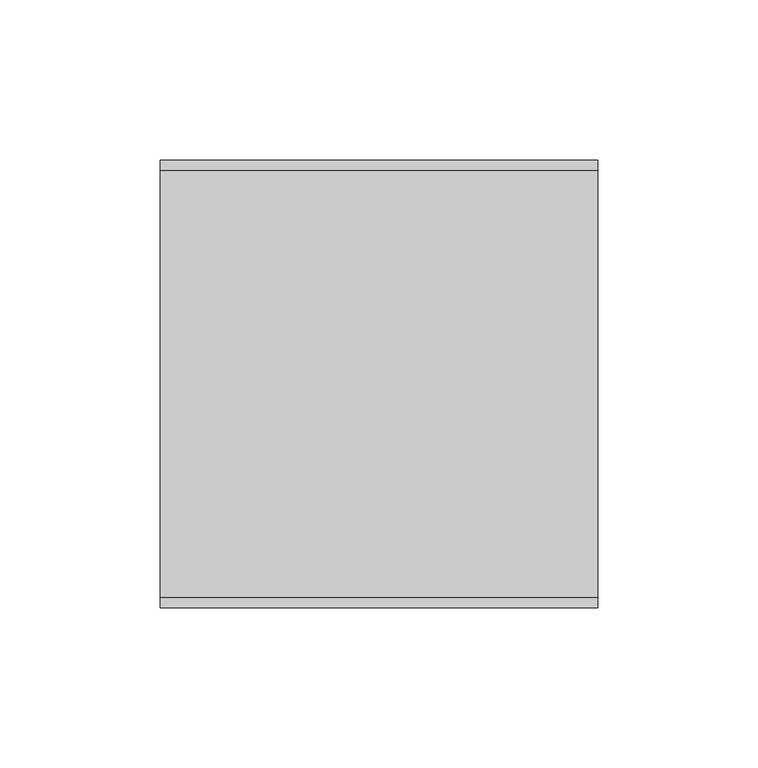
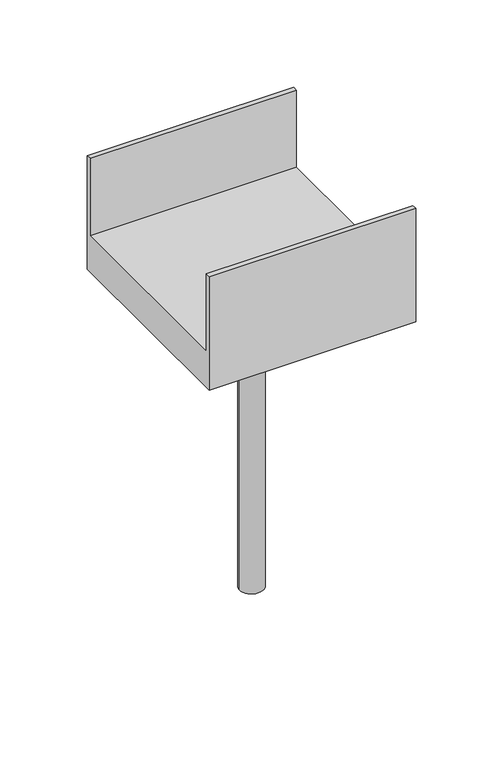
"""IFC4 building model written with IfcOpenShell, lengths in millimetres: fastener geometry."""

import ifcopenshell
import ifcopenshell.guid

model = None  # the IFC model being written
_history = None  # IfcOwnerHistory: only IFC2X3 demands one
_inside = {}  # id of a spatial element -> (the spatial element, [elements in it])
_under = {}  # id of a project, library or spatial element -> (it, [spatial elements below it])
_declared = {}  # id of a project -> (the project, [libraries it declares])
_typed = {}  # id of a type object -> (the type object, [elements of that type])
_made_of = {}  # id of a material, layer set ... -> (it, [elements and type objects made of it])


def new_model(schema):
    """Start an empty IFC model of exactly this schema.

    Asked for "IFC4X3", IfcOpenShell would pick the latest addendum, in which some entities
    have other attributes; the version numbers below select the first issue.
    IFC2X3 requires an IfcOwnerHistory on every rooted entity: one is made here for all.
    """
    global model, _history
    if schema == "IFC4X3":
        model = ifcopenshell.file(schema_version=(4, 3, 0, 0))
    else:
        model = ifcopenshell.file(schema=schema)
    _inside.clear()
    _under.clear()
    _declared.clear()
    _typed.clear()
    _made_of.clear()
    _history = None
    if model.schema == "IFC2X3":
        org = make("IfcOrganization", Name="unknown")
        user = make(
            "IfcPersonAndOrganization",
            ThePerson=make("IfcPerson", FamilyName="unknown"),
            TheOrganization=org,
        )
        app = make(
            "IfcApplication",
            ApplicationDeveloper=org,
            Version="unknown",
            ApplicationFullName="unknown",
            ApplicationIdentifier="unknown",
        )
        _history = make(
            "IfcOwnerHistory",
            OwningUser=user,
            OwningApplication=app,
            ChangeAction="ADDED",
            CreationDate=0,
        )
    return model


def make(cls, **values):
    """One entity of the class cls with the attributes given. An attribute that is None is left unset."""
    return model.create_entity(
        cls, **{name: value for name, value in values.items() if value is not None}
    )


def rooted(cls, **values):
    """An entity with a GlobalId (a new one), such as an element, a storey or a relation."""
    return make(cls, GlobalId=ifcopenshell.guid.new(), OwnerHistory=_history, **values)


def si_unit(unit_type, name, prefix=None):
    """IfcSIUnit, for example si_unit("LENGTHUNIT", "METRE", prefix="MILLI")."""
    return make("IfcSIUnit", UnitType=unit_type, Prefix=prefix, Name=name)


def assignment(units):
    """IfcUnitAssignment: the units of a project."""
    return None if units is None else make("IfcUnitAssignment", Units=units)


def point(xyz):
    """IfcCartesianPoint."""
    return None if xyz is None else make("IfcCartesianPoint", Coordinates=xyz)


def direction(xyz):
    """IfcDirection."""
    return None if xyz is None else make("IfcDirection", DirectionRatios=xyz)


def frame(location, z_axis=None, x_axis=None):
    """IfcAxis2Placement3D, a coordinate frame: its origin and axes. An axis left out is left unset."""
    return make(
        "IfcAxis2Placement3D",
        Location=point(location),
        Axis=direction(z_axis),
        RefDirection=direction(x_axis),
    )


def frame_2d(location, x_axis=None):
    """IfcAxis2Placement2D, a coordinate frame in the plane: its origin and x axis."""
    return make(
        "IfcAxis2Placement2D", Location=point(location), RefDirection=direction(x_axis)
    )


def origin():
    """The frame at (0, 0, 0) with its axes left unset."""
    return frame((0.0, 0.0, 0.0))


def origin_with_axes():
    """The frame at (0, 0, 0) with the z axis (0, 0, 1) and the x axis (1, 0, 0) written out."""
    return frame((0.0, 0.0, 0.0), z_axis=(0.0, 0.0, 1.0), x_axis=(1.0, 0.0, 0.0))


def origin_2d():
    """The frame at (0, 0) in the plane with its x axis left unset."""
    return frame_2d((0.0, 0.0))


def place(relative_to, where):
    """IfcLocalPlacement: puts the frame where relative to a parent placement (None: the world)."""
    return make(
        "IfcLocalPlacement", PlacementRelTo=relative_to, RelativePlacement=where
    )


def context(
    kind, dimensions, precision=None, world=None, true_north=None, identifier=None
):
    """IfcGeometricRepresentationContext, for example the 3D "Model" context."""
    return make(
        "IfcGeometricRepresentationContext",
        ContextIdentifier=identifier,
        ContextType=kind,
        CoordinateSpaceDimension=dimensions,
        Precision=precision,
        WorldCoordinateSystem=world,
        TrueNorth=true_north,
    )


def project(units=None, contexts=None):
    """IfcProject with its units and contexts."""
    return rooted(
        "IfcProject",
        Name="project",
        RepresentationContexts=contexts,
        UnitsInContext=assignment(units),
    )


def spatial(cls, under=None, at=None, **own):
    """A site, building, storey or space (cls), placed at a placement, below another one or the project."""
    s = rooted(cls, ObjectPlacement=at, **own)
    if under is not None:
        _under.setdefault(under.id(), (under, []))[1].append(s)
    return s


def polyline(points):
    """IfcPolyline through the points."""
    return make("IfcPolyline", Points=[point(p) for p in points])


def circle_curve(where, radius):
    """IfcCircle in the frame where."""
    return make("IfcCircle", Position=where, Radius=radius)


def trimmed(basis, trim1, trim2, sense, master):
    """IfcTrimmedCurve: the piece of a basis curve between two trims."""
    return make(
        "IfcTrimmedCurve",
        BasisCurve=basis,
        Trim1=trim1,
        Trim2=trim2,
        SenseAgreement=sense,
        MasterRepresentation=master,
    )


def segment(curve, same_sense, transition):
    """IfcCompositeCurveSegment."""
    return make(
        "IfcCompositeCurveSegment",
        Transition=transition,
        SameSense=same_sense,
        ParentCurve=curve,
    )


def composite_curve(segments, self_intersect=None):
    """IfcCompositeCurve: segments joined end to end."""
    return make("IfcCompositeCurve", Segments=segments, SelfIntersect=self_intersect)


def outline(outer, holes=None, kind="AREA"):
    """IfcArbitraryClosedProfileDef: a profile drawn as a closed curve; with holes, ...WithVoids."""
    if holes is None:
        return make("IfcArbitraryClosedProfileDef", ProfileType=kind, OuterCurve=outer)
    return make(
        "IfcArbitraryProfileDefWithVoids",
        ProfileType=kind,
        OuterCurve=outer,
        InnerCurves=holes,
    )


def extrude(swept, where, along, depth):
    """IfcExtrudedAreaSolid: the profile swept, set in the frame where, extruded along a direction by depth."""
    return make(
        "IfcExtrudedAreaSolid",
        SweptArea=swept,
        Position=where,
        ExtrudedDirection=direction(along),
        Depth=depth,
    )


def shape(context_of_items, identifier, shape_type, items):
    """IfcShapeRepresentation: the items that make up one representation, for example the "Body"."""
    return make(
        "IfcShapeRepresentation",
        ContextOfItems=context_of_items,
        RepresentationIdentifier=identifier,
        RepresentationType=shape_type,
        Items=items,
    )


def source(mapping_origin, context_of_items, identifier, shape_type, items):
    """IfcRepresentationMap: a shape defined once, which mapped items show again and again."""
    return make(
        "IfcRepresentationMap",
        MappingOrigin=mapping_origin,
        MappedRepresentation=shape(context_of_items, identifier, shape_type, items),
    )


def transform(
    local_origin,
    x_axis=None,
    y_axis=None,
    z_axis=None,
    scale=None,
    scale2=None,
    scale3=None,
    uniform=True,
):
    """IfcCartesianTransformationOperator3D, or its non-uniform kind. x_axis, y_axis, z_axis: its Axis1, 2, 3."""
    if uniform:
        return make(
            "IfcCartesianTransformationOperator3D",
            Axis1=direction(x_axis),
            Axis2=direction(y_axis),
            LocalOrigin=point(local_origin),
            Scale=scale,
            Axis3=direction(z_axis),
        )
    return make(
        "IfcCartesianTransformationOperator3DnonUniform",
        Axis1=direction(x_axis),
        Axis2=direction(y_axis),
        LocalOrigin=point(local_origin),
        Scale=scale,
        Axis3=direction(z_axis),
        Scale2=scale2,
        Scale3=scale3,
    )


def mapped(mapping_source, mapping_target):
    """IfcMappedItem: shows the shape of a source again, moved by a transform."""
    return make(
        "IfcMappedItem", MappingSource=mapping_source, MappingTarget=mapping_target
    )


def made_of(thing, what):
    """Note that an element or type object is made of a material, layer set ...; save() writes the relation."""
    if what is not None:
        _made_of.setdefault(what.id(), (what, []))[1].append(thing)
    return thing


def element(
    cls,
    number,
    at=None,
    inside=None,
    cuts=None,
    type_object=None,
    material=None,
    context=None,
    identifier="Body",
    shape_type=None,
    held_by="IfcProductDefinitionShape",
    body=None,
    shapes=None,
    **own,
):
    """One element of the class cls, such as IfcWall. Its Tag is "e" and its number.

    at: its placement. inside: the storey or other place that contains it. cuts: it is an
    opening in that element (IfcRelVoidsElement). A single representation is given by context,
    identifier, shape_type and body (its items); several are given by shapes. held_by: the class
    of the entity that holds the representations. save() writes the other relations.
    """
    e = rooted(cls, Tag="e%d" % number, ObjectPlacement=at, **own)
    if body is not None:
        shapes = [shape(context, identifier, shape_type, body)]
    if shapes is not None:
        e.Representation = make(held_by, Representations=shapes)
    if inside is not None:
        _inside.setdefault(inside.id(), (inside, []))[1].append(e)
    if cuts is not None:
        rooted(
            "IfcRelVoidsElement", RelatingBuildingElement=cuts, RelatedOpeningElement=e
        )
    if type_object is not None:
        _typed.setdefault(type_object.id(), (type_object, []))[1].append(e)
    return made_of(e, material)


def aggregate(whole, parts):
    """IfcRelAggregates: a whole, such as a stair, and the parts it consists of."""
    return rooted("IfcRelAggregates", RelatingObject=whole, RelatedObjects=parts)


def save(model, path):
    """Write the relations noted so far, then the file.

    IfcRelAggregates (storeys below a building ...), IfcRelContainedInSpatialStructure (elements
    in a storey), IfcRelDefinesByType, IfcRelAssociatesMaterial and IfcRelDeclares: one each for
    every whole, place, type object, material and project.
    """
    for whole, parts in _under.values():
        aggregate(whole, parts)
    for where, things in _inside.values():
        rooted(
            "IfcRelContainedInSpatialStructure",
            RelatedElements=things,
            RelatingStructure=where,
        )
    for kind, things in _typed.values():
        rooted("IfcRelDefinesByType", RelatedObjects=things, RelatingType=kind)
    for what, things in _made_of.values():
        rooted("IfcRelAssociatesMaterial", RelatedObjects=things, RelatingMaterial=what)
    for by, libraries in _declared.values():
        rooted("IfcRelDeclares", RelatingContext=by, RelatedDefinitions=libraries)
    model.write(path)


def fastener_d5b4f6b8(model_context):
    return source(origin(), model_context, "Body", "SweptSolid", [
        extrude(outline(composite_curve([segment(trimmed(circle_curve(origin_2d(), 7.9375), [point((-7.9375, 0.0))], [point((7.9375, 0.0))], False, "CARTESIAN"), True, "CONTINUOUS"), segment(trimmed(circle_curve(origin_2d(), 7.9375), [point((7.9375, 0.0))], [point((-7.9375, 0.0))], False, "CARTESIAN"), True, "CONTINUOUS")], self_intersect=False)), frame((0.0, 0.0, -203.2), z_axis=(0.0, 0.0, 1.0), x_axis=(1.0, 0.0, 0.0)), (0.0, 0.0, 1.0), 203.2),
        extrude(outline(polyline([(-11.90625, 6.8740766), (0.0, 13.7481533), (11.90625, 6.8740766), (11.90625, -6.8740766), (0.0, -13.7481533), (-11.90625, -6.8740766), (-11.90625, 6.8740766)])), origin_with_axes(), (0.0, 0.0, 1.0), 11.2117187),
        extrude(outline(polyline([(-69.85, 79.375), (-66.675, 79.375), (-66.675, 25.4), (66.675, 25.4), (66.675, 79.375), (69.85, 79.375), (69.85, 0.0), (-69.85, 0.0), (-69.85, 79.375)])), frame((-68.2625, 0.0, 0.0), z_axis=(1.0, 0.0, 0.0), x_axis=(0.0, 1.0, 0.0)), (0.0, 0.0, 1.0), 136.525),
    ])


if __name__ == "__main__":
    model = new_model("IFC4")
    model_context = context("Model", 3, world=origin())
    ifc_project = project(units=[si_unit("LENGTHUNIT", "METRE", prefix="MILLI")], contexts=[model_context])
    site = spatial("IfcSite", under=ifc_project)
    building = spatial("IfcBuilding", under=site)
    placement = place(None, origin())
    fastener_shape = fastener_d5b4f6b8(model_context)
    element("IfcFastener", 1, ObjectType="SIMPSON - ABA- POST BASE : SIMPSON - ABA66Z W/ 5/8\"X8\" ANCHOR BOLT W/ NON-SHRINK GROUT AT BASE", at=placement, inside=building, context=model_context, shape_type="MappedRepresentation", body=[
        mapped(fastener_shape, transform((0.0, 0.0, 0.0), x_axis=(1.0, 0.0, 0.0), y_axis=(0.0, 1.0, 0.0), z_axis=(0.0, 0.0, 1.0))),
    ])
    save(model, "model.ifc")

# Revit data of these elements
# Type "SIMPSON - ABA- POST BASE : SIMPSON - ABA66Z W/ 5/8\"X8\" ANCHOR BOLT W/ NON-SHRINK GROUT AT BASE"
#   L = 0' - 3"
#   Hole Radius = 0' - 0 3/8"
#   D4 = 0' - 5"
#   D2 = 0' - 5"
#   D1 = 0' - 1 1/2"
#   D3 = 0' - 2 3/4"
#   Ga. = 0' - 0 61/256"
#   W1 & W2 = 0' - 4 1/4"
#   Default Elevation = 4' - 0"
#   Bolt Visibility - 3B = no
#   Bolt Visibility - 3A = no
#   Bolt Visibility - 2B = no
#   Bolt Visibility - 2A = no
#   Bolt Visibility - 1B = no
#   Bolt Visibility - 1A = yes
#   Bolt Visibility = yes
#   Material = ABA66Z W/ 5/8"X8" ANCHOR BOLT W/ NON-SHRINK GROUT AT BASE
#   Bolt Size = element 1605874
#   URL = ""
# Element 1 (IfcFastener, "SIMPSON - ABA- POST BASE : SIMPSON - ABA66Z W/ 5/8\"X8\" ANCHOR BOLT W/ NON-SHRINK GROUT AT BASE")
#   Materials on its faces: "1\" GALV. LAG BOLT (LENGTH = 1/2\" SHY OF GLULAM DEPTH) -  (GALV. THRU BOLT IF PLATE ON OPP. SIDE OF STRUCT MEMBER)", "ABA66Z W/ 5/8\"X8\" ANCHOR BOLT W/ NON-SHRINK GROUT AT BASE"
# Materials
#   "ABA66Z W/ 5/8\"X8\" ANCHOR BOLT W/ NON-SHRINK GROUT AT BASE": class "Generic", colour RGB 232 232 232, transparency 0, Cost = 0
#   "1\" GALV. LAG BOLT (LENGTH = 1/2\" SHY OF GLULAM DEPTH) -  (GALV. THRU BOLT IF PLATE ON OPP. SIDE OF STRUCT MEMBER)": class "Generic", colour RGB 120 120 120, transparency 0, Cost = 0
